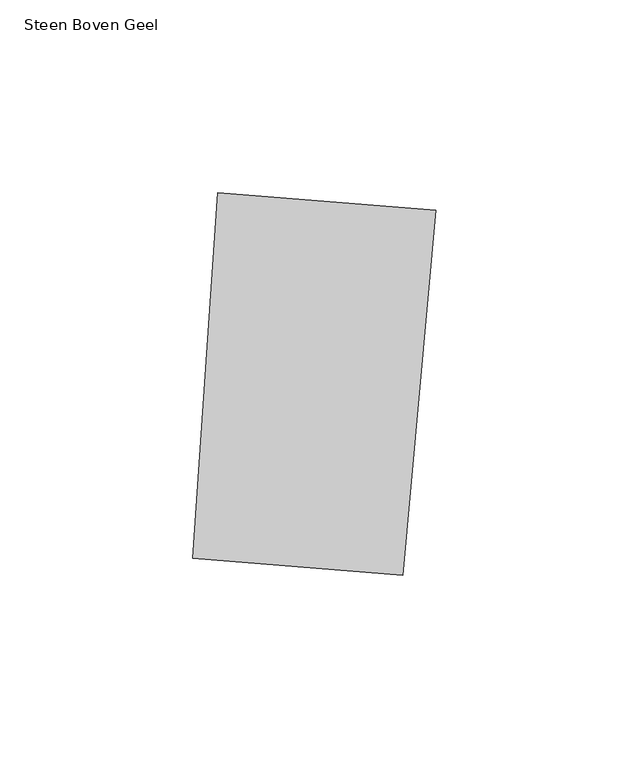
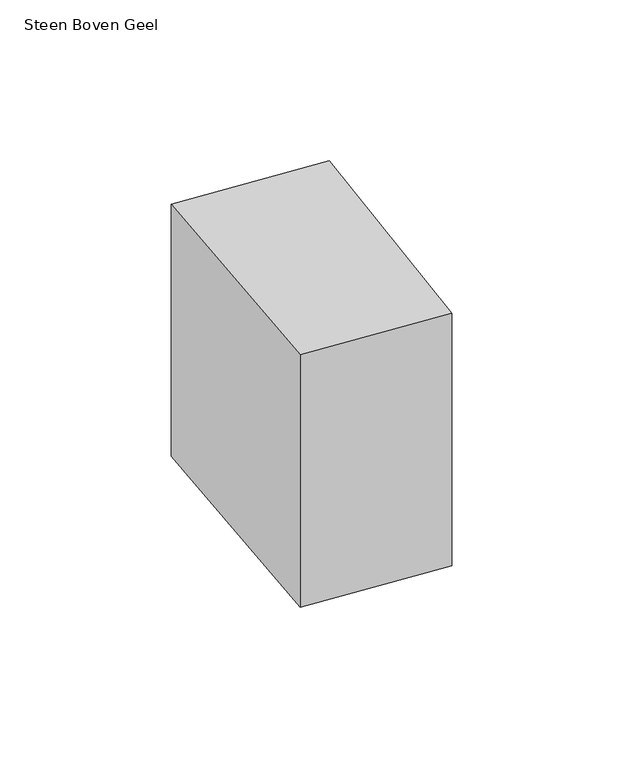
"""IFC4 building model written with IfcOpenShell, lengths in millimetres: proxy geometry, 00_GMA_steen_versie_4 : Steen Boven Geel."""

from ifc_helpers import new_model, si_unit, origin, origin_with_axes, place, context, project, spatial, polyline, outline, extrude, source, transform, mapped, element, save


def steen_boven_geel_941cf55b(model_context):
    return source(origin(), model_context, "Body", "SweptSolid", [
        extrude(outline(polyline([(105.0889481, 118.7912944), (96.5008029, 24.1740834), (42.1171699, 28.5017098), (48.6008496, 123.2863855), (105.0889481, 118.7912944)])), origin_with_axes(), (0.0, 0.0, 1.0), 100.0),
    ])


if __name__ == "__main__":
    model = new_model("IFC4")
    model_context = context("Model", 3, world=origin())
    ifc_project = project(units=[si_unit("LENGTHUNIT", "METRE", prefix="MILLI")], contexts=[model_context])
    site = spatial("IfcSite", under=ifc_project)
    building = spatial("IfcBuilding", under=site)
    placement = place(None, origin())
    steen_boven_geel_shape = steen_boven_geel_941cf55b(model_context)
    element("IfcBuildingElementProxy", 1, Name="00_GMA_steen_versie_4 : Steen Boven Geel", ObjectType="00_GMA_steen_versie_4 : Steen Boven Geel", at=placement, inside=building, context=model_context, shape_type="MappedRepresentation", body=[
        mapped(steen_boven_geel_shape, transform((0.0, 0.0, 0.0), x_axis=(1.0, 0.0, 0.0), y_axis=(0.0, 1.0, 0.0), z_axis=(0.0, 0.0, 1.0))),
    ])
    save(model, "model.ifc")

# Revit data of these elements
# Type "00_GMA_steen_versie_4 : Steen Boven Geel"
#   StootVoegHalfBoven [instance default] = 5 mm
#   StootVoegHalf [instance default] = 5 mm
#   StootVoegBreedteOnder = 10 mm
#   StootVoegBreedteBoven = 10 mm
#   Steendikte = 100 mm
#   LintVoegOnderHalf = 5 mm
#   LintVoegOnder = 10 mm
#   LintVoegBovenHalf = 0 mm
#   LintVoegBoven = 0 mm
#   materiaal = 21_steen_geel
#   MateriaalVoeg = none
#   Default Elevation = 0
# Element 1 (IfcBuildingElementProxy, "00_GMA_steen_versie_4 : Steen Boven Geel")
#   Materials on its faces: "21_steen_geel"
# Materials
#   "21_steen_geel": class "Unassigned", colour RGB 202 202 0, transparency 0, Cost = 0
